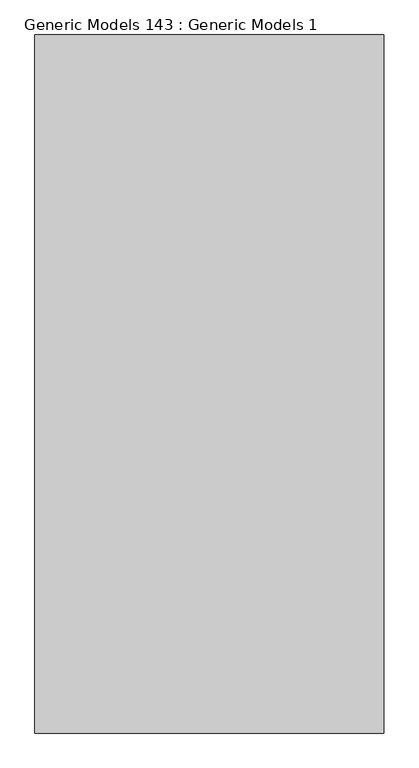
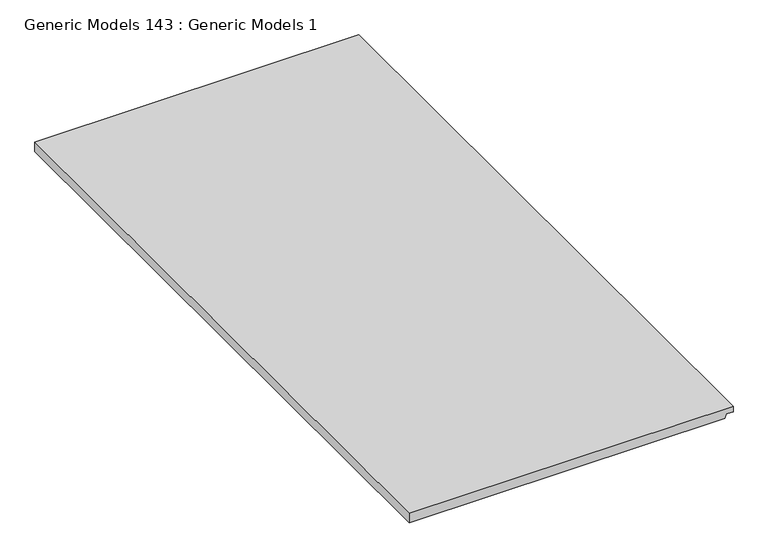
"""IFC4 building model written with IfcOpenShell, lengths in millimetres: proxy geometry, Generic Models 143 : Generic Models 1."""

from ifc_helpers import new_model, si_unit, frame, origin, place, context, project, spatial, polyline, outline, extrude, source, transform, mapped, element, save


def generic_models_143_generic_models_1_b299bc08(model_context):
    return source(origin(), model_context, "Body", "SweptSolid", [
        extrude(outline(polyline([(102.9070404, 49680.8980231), (102.9070404, 49071.2980231), (83.8570404, 49071.2980231), (83.8570404, 49665.3090094), (91.7945404, 49668.1980231), (91.7945404, 49680.8980231), (102.9070404, 49680.8980231)])), frame((0.0, 0.0, 0.0), z_axis=(0.0, 1.0, 0.0), x_axis=(0.0, 0.0, 1.0)), (0.0, 0.0, 1.0), 1219.2),
    ])


if __name__ == "__main__":
    model = new_model("IFC4")
    model_context = context("Model", 3, world=origin())
    ifc_project = project(units=[si_unit("LENGTHUNIT", "METRE", prefix="MILLI")], contexts=[model_context])
    site = spatial("IfcSite", under=ifc_project)
    building = spatial("IfcBuilding", under=site)
    placement = place(None, origin())
    generic_models_143_generic_models_1_shape = generic_models_143_generic_models_1_b299bc08(model_context)
    element("IfcBuildingElementProxy", 1, Name="Generic Models 143 : Generic Models 1", ObjectType="Generic Models 143 : Generic Models 1", at=placement, inside=building, context=model_context, shape_type="MappedRepresentation", body=[
        mapped(generic_models_143_generic_models_1_shape, transform((0.0, 0.0, 0.0), x_axis=(1.0, 0.0, 0.0), y_axis=(0.0, 1.0, 0.0), z_axis=(0.0, 0.0, 1.0))),
    ])
    save(model, "model.ifc")

# Revit data of these elements
# Element 1 (IfcBuildingElementProxy, "Generic Models 143 : Generic Models 1")
#   Materials on its faces: "EXISTING ACT CEILING"
# Materials
#   "EXISTING ACT CEILING": class "Generic", colour RGB 255 255 255, transparency 0, Cost = 0
